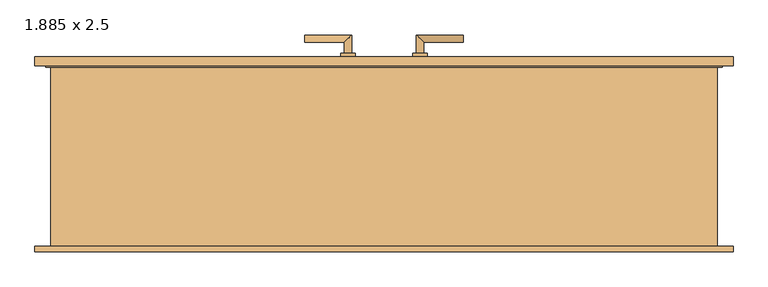
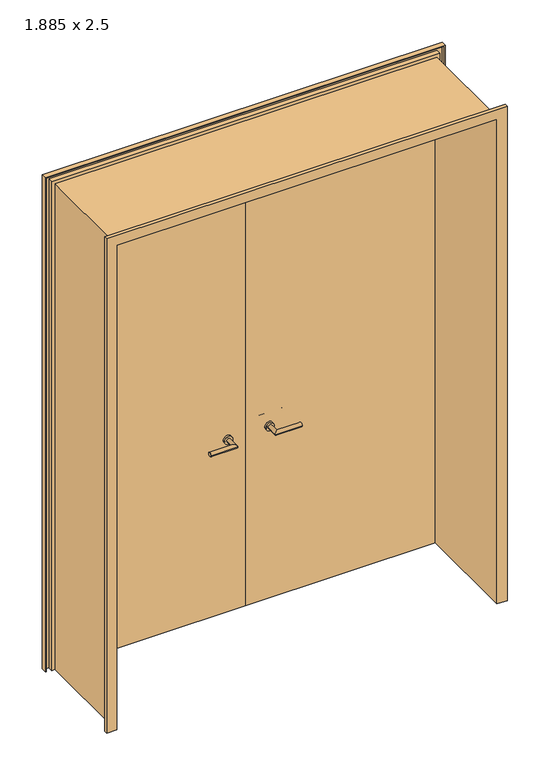
"""IFC4 building model written with IfcOpenShell, lengths in millimetres: door geometry, Drehflügel 2-flg - Stahlzarge : 1.885 x 2.5."""

from ifc_helpers import new_model, si_unit, point, frame, frame_2d, origin, place, context, project, spatial, polyline, circle_curve, ellipse_curve, trimmed, segment, composite_curve, outline, extrude, faceted_brep, source, transform, mapped, element, save
from ifc_brep_helpers import plane_surface, cylinder_surface, advanced_brep


def door_1_885_x_2_5_dd39479c(model_context):
    return source(origin(), model_context, "Body", "SolidModel", [
        advanced_brep(
        [(-90.0, 239.4346141, 901.0), (-110.0, 239.4346141, 901.0), (-110.0, 189.4346141, 901.0), (-90.0, 169.4346141, 901.0), (-220.0, 169.4346141, 901.0), (-220.0, 189.4346141, 901.0)],
        [
            (0, 1, circle_curve(frame((-100.0, 239.4346141, 901.0), z_axis=(0.0, 1.0, 0.0), x_axis=(-1.0, 0.0, 0.0)), 10.0)),
            (1, 0, circle_curve(frame((-100.0, 239.4346141, 901.0), z_axis=(0.0, 1.0, 0.0), x_axis=(-1.0, 0.0, 0.0)), 10.0)),
            (1, 2),
            (2, 3, ellipse_curve(frame((-100.0, 179.4346141, 901.0), z_axis=(0.7071067811865385, 0.7071067811865565, 0.0), x_axis=(-0.7071067811865563, 0.7071067811865386, 0.0)), 14.1421356, 10.0)),
            (3, 0),
            (3, 2, ellipse_curve(frame((-100.0, 179.4346141, 901.0), z_axis=(0.7071067811865385, 0.7071067811865565, 0.0), x_axis=(-0.7071067811865563, 0.7071067811865386, 0.0)), 14.1421356, 10.0)),
            (4, 5, circle_curve(frame((-220.0, 179.4346141, 901.0), z_axis=(-1.0, 0.0, 0.0), x_axis=(0.0, 1.0, 0.0)), 10.0)),
            (5, 4, circle_curve(frame((-220.0, 179.4346141, 901.0), z_axis=(-1.0, 0.0, 0.0), x_axis=(0.0, 1.0, 0.0)), 10.0)),
            (2, 5),
            (4, 3),
        ],
        [
            plane_surface(frame((-100.0, 239.4346141, -386.7526403), z_axis=(0.0, 1.0, 0.0), x_axis=(0.0, 0.0, 1.0))),
            cylinder_surface(frame((-100.0, 239.4346141, 901.0), z_axis=(0.0, 1.0, 0.0), x_axis=(-1.0, 0.0, 0.0)), 10.0),
            plane_surface(frame((-220.0, 179.4346141, -386.7526403), z_axis=(-1.0, 0.0, 0.0), x_axis=(0.0, 0.0, 1.0))),
            cylinder_surface(frame((-100.0, 179.4346141, 901.0), z_axis=(1.0, 0.0, 0.0), x_axis=(0.0, 1.0, 0.0)), 10.0),
        ],
        [
            (0, [[1, 2]]),
            (1, [[3, 4, 5, -2]]),
            (1, [[-5, 6, -3, -1]]),
            (2, [[7, 8]]),
            (3, [[9, -7, 10, -4]]),
            (3, [[-10, -8, -9, -6]]),
        ],
    ),
        advanced_brep(
        [(-110.0, 299.4346141, 901.0), (-90.0, 299.4346141, 901.0), (-90.0, 349.4346141, 901.0), (-110.0, 329.4346141, 901.0), (-220.0, 329.4346141, 901.0), (-220.0, 349.4346141, 901.0)],
        [
            (0, 1, circle_curve(frame((-100.0, 299.4346141, 901.0), z_axis=(0.0, -1.0, 0.0), x_axis=(1.0, 0.0, 0.0)), 10.0)),
            (1, 0, circle_curve(frame((-100.0, 299.4346141, 901.0), z_axis=(0.0, -1.0, 0.0), x_axis=(1.0, 0.0, 0.0)), 10.0)),
            (1, 2),
            (2, 3, ellipse_curve(frame((-100.0, 339.4346141, 901.0), z_axis=(0.7071067811865475, -0.7071067811865475, 0.0), x_axis=(-0.7071067811865474, -0.7071067811865476, 0.0)), 14.1421356, 10.0)),
            (3, 0),
            (3, 2, ellipse_curve(frame((-100.0, 339.4346141, 901.0), z_axis=(0.7071067811865475, -0.7071067811865475, 0.0), x_axis=(-0.7071067811865474, -0.7071067811865476, 0.0)), 14.1421356, 10.0)),
            (4, 5, circle_curve(frame((-220.0, 339.4346141, 901.0), z_axis=(-1.0, 0.0, 0.0), x_axis=(0.0, 1.0, 0.0)), 10.0)),
            (5, 4, circle_curve(frame((-220.0, 339.4346141, 901.0), z_axis=(-1.0, 0.0, 0.0), x_axis=(0.0, 1.0, 0.0)), 10.0)),
            (2, 5),
            (4, 3),
        ],
        [
            plane_surface(frame((-100.0, 299.4346141, -386.7526403), z_axis=(0.0, -1.0, 0.0), x_axis=(0.0, 0.0, 1.0))),
            cylinder_surface(frame((-100.0, 299.4346141, 901.0), z_axis=(0.0, -1.0, 0.0), x_axis=(1.0, 0.0, 0.0)), 10.0),
            plane_surface(frame((-220.0, 339.4346141, -386.7526403), z_axis=(-1.0, 0.0, 0.0), x_axis=(0.0, 0.0, 1.0))),
            cylinder_surface(frame((-100.0, 339.4346141, 901.0), z_axis=(1.0, 0.0, 0.0), x_axis=(0.0, 1.0, 0.0)), 10.0),
        ],
        [
            (0, [[1, 2]]),
            (1, [[3, 4, 5, -2]]),
            (1, [[-5, 6, -3, -1]]),
            (2, [[7, 8]]),
            (3, [[9, -7, 10, -4]]),
            (3, [[-10, -8, -9, -6]]),
        ],
    ),
        extrude(outline(composite_curve([segment(trimmed(circle_curve(frame_2d((901.0, -100.0)), 20.0), [point((901.0, -80.0))], [point((901.0, -120.0))], False, "CARTESIAN"), True, "CONTINUOUS"), segment(trimmed(circle_curve(frame_2d((901.0, -100.0)), 20.0), [point((901.0, -120.0))], [point((901.0, -80.0))], False, "CARTESIAN"), True, "CONTINUOUS")], self_intersect=False)), frame((0.0, 229.4346141, 0.0), z_axis=(0.0, 1.0, 0.0), x_axis=(0.0, 0.0, 1.0)), (0.0, 0.0, 1.0), 10.0),
        extrude(outline(composite_curve([segment(trimmed(circle_curve(frame_2d((901.0, -100.0)), 20.0), [point((901.0, -80.0))], [point((901.0, -120.0))], False, "CARTESIAN"), True, "CONTINUOUS"), segment(trimmed(circle_curve(frame_2d((901.0, -100.0)), 20.0), [point((901.0, -120.0))], [point((901.0, -80.0))], False, "CARTESIAN"), True, "CONTINUOUS")], self_intersect=False)), frame((0.0, 289.4346141, 0.0), z_axis=(0.0, 1.0, 0.0), x_axis=(0.0, 0.0, 1.0)), (0.0, 0.0, 1.0), 10.0),
        advanced_brep(
        [(90.0, 239.4346141, 901.0), (110.0, 239.4346141, 901.0), (90.0, 169.4346141, 901.0), (110.0, 189.4346141, 901.0), (220.0, 169.4346141, 901.0), (220.0, 189.4346141, 901.0)],
        [
            (0, 1, circle_curve(frame((100.0, 239.4346141, 901.0), z_axis=(0.0, 1.0, 0.0), x_axis=(1.0, 0.0, 0.0)), 10.0)),
            (1, 0, circle_curve(frame((100.0, 239.4346141, 901.0), z_axis=(0.0, 1.0, 0.0), x_axis=(1.0, 0.0, 0.0)), 10.0)),
            (0, 2),
            (2, 3, ellipse_curve(frame((100.0, 179.4346141, 901.0), z_axis=(-0.7071067811865385, 0.7071067811865565, 0.0), x_axis=(0.7071067811865563, 0.7071067811865386, 0.0)), 14.1421356, 10.0)),
            (3, 1),
            (3, 2, ellipse_curve(frame((100.0, 179.4346141, 901.0), z_axis=(-0.7071067811865385, 0.7071067811865565, 0.0), x_axis=(0.7071067811865563, 0.7071067811865386, 0.0)), 14.1421356, 10.0)),
            (4, 5, circle_curve(frame((220.0, 179.4346141, 901.0), z_axis=(1.0, 0.0, 0.0), x_axis=(0.0, 1.0, 0.0)), 10.0)),
            (5, 4, circle_curve(frame((220.0, 179.4346141, 901.0), z_axis=(1.0, 0.0, 0.0), x_axis=(0.0, 1.0, 0.0)), 10.0)),
            (2, 4),
            (5, 3),
        ],
        [
            plane_surface(frame((100.0, 239.4346141, -386.7526403), z_axis=(0.0, 1.0, 0.0), x_axis=(0.0, 0.0, 1.0))),
            cylinder_surface(frame((100.0, 239.4346141, 901.0), z_axis=(0.0, 1.0, 0.0), x_axis=(1.0, 0.0, 0.0)), 10.0),
            plane_surface(frame((220.0, 179.4346141, -386.7526403), z_axis=(1.0, 0.0, 0.0), x_axis=(0.0, 0.0, 1.0))),
            cylinder_surface(frame((100.0, 179.4346141, 901.0), z_axis=(-1.0, 0.0, 0.0), x_axis=(0.0, 1.0, 0.0)), 10.0),
        ],
        [
            (0, [[1, 2]]),
            (1, [[-1, 3, 4, 5]]),
            (1, [[-2, -5, 6, -3]]),
            (2, [[7, 8]]),
            (3, [[-4, 9, -8, 10]]),
            (3, [[-6, -10, -7, -9]]),
        ],
    ),
        advanced_brep(
        [(110.0, 299.4346141, 901.0), (90.0, 299.4346141, 901.0), (110.0, 329.4346141, 901.0), (90.0, 349.4346141, 901.0), (220.0, 329.4346141, 901.0), (220.0, 349.4346141, 901.0)],
        [
            (0, 1, circle_curve(frame((100.0, 299.4346141, 901.0), z_axis=(0.0, -1.0, 0.0), x_axis=(-1.0, 0.0, 0.0)), 10.0)),
            (1, 0, circle_curve(frame((100.0, 299.4346141, 901.0), z_axis=(0.0, -1.0, 0.0), x_axis=(-1.0, 0.0, 0.0)), 10.0)),
            (0, 2),
            (2, 3, ellipse_curve(frame((100.0, 339.4346141, 901.0), z_axis=(-0.7071067811865475, -0.7071067811865475, 0.0), x_axis=(0.7071067811865474, -0.7071067811865476, 0.0)), 14.1421356, 10.0)),
            (3, 1),
            (3, 2, ellipse_curve(frame((100.0, 339.4346141, 901.0), z_axis=(-0.7071067811865475, -0.7071067811865475, 0.0), x_axis=(0.7071067811865474, -0.7071067811865476, 0.0)), 14.1421356, 10.0)),
            (4, 5, circle_curve(frame((220.0, 339.4346141, 901.0), z_axis=(1.0, 0.0, 0.0), x_axis=(0.0, 1.0, 0.0)), 10.0)),
            (5, 4, circle_curve(frame((220.0, 339.4346141, 901.0), z_axis=(1.0, 0.0, 0.0), x_axis=(0.0, 1.0, 0.0)), 10.0)),
            (2, 4),
            (5, 3),
        ],
        [
            plane_surface(frame((100.0, 299.4346141, -386.7526403), z_axis=(0.0, -1.0, 0.0), x_axis=(0.0, 0.0, 1.0))),
            cylinder_surface(frame((100.0, 299.4346141, 901.0), z_axis=(0.0, -1.0, 0.0), x_axis=(-1.0, 0.0, 0.0)), 10.0),
            plane_surface(frame((220.0, 339.4346141, -386.7526403), z_axis=(1.0, 0.0, 0.0), x_axis=(0.0, 0.0, 1.0))),
            cylinder_surface(frame((100.0, 339.4346141, 901.0), z_axis=(-1.0, 0.0, 0.0), x_axis=(0.0, 1.0, 0.0)), 10.0),
        ],
        [
            (0, [[1, 2]]),
            (1, [[-1, 3, 4, 5]]),
            (1, [[-2, -5, 6, -3]]),
            (2, [[7, 8]]),
            (3, [[-4, 9, -8, 10]]),
            (3, [[-6, -10, -7, -9]]),
        ],
    ),
        extrude(outline(composite_curve([segment(trimmed(circle_curve(frame_2d((901.0, 100.0)), 20.0), [point((901.0, 80.0))], [point((901.0, 120.0))], False, "CARTESIAN"), True, "CONTINUOUS"), segment(trimmed(circle_curve(frame_2d((901.0, 100.0)), 20.0), [point((901.0, 120.0))], [point((901.0, 80.0))], False, "CARTESIAN"), True, "CONTINUOUS")], self_intersect=False)), frame((0.0, 229.4346141, 0.0), z_axis=(0.0, 1.0, 0.0), x_axis=(0.0, 0.0, 1.0)), (0.0, 0.0, 1.0), 10.0),
        extrude(outline(composite_curve([segment(trimmed(circle_curve(frame_2d((901.0, 100.0)), 20.0), [point((901.0, 80.0))], [point((901.0, 120.0))], False, "CARTESIAN"), True, "CONTINUOUS"), segment(trimmed(circle_curve(frame_2d((901.0, 100.0)), 20.0), [point((901.0, 120.0))], [point((901.0, 80.0))], False, "CARTESIAN"), True, "CONTINUOUS")], self_intersect=False)), frame((0.0, 289.4346141, 0.0), z_axis=(0.0, 1.0, 0.0), x_axis=(0.0, 0.0, 1.0)), (0.0, 0.0, 1.0), 10.0),
        extrude(outline(polyline([(0.0, 264.4346141), (-932.5, 264.4346141), (-932.5, 289.4346141), (0.0, 289.4346141), (0.0, 264.4346141)])), frame((0.0, 0.0, 1.0), z_axis=(0.0, 0.0, 1.0), x_axis=(1.0, 0.0, 0.0)), (0.0, 0.0, 1.0), 2490.0),
        extrude(outline(polyline([(932.5, 264.4346141), (0.0, 264.4346141), (0.0, 289.4346141), (932.5, 289.4346141), (932.5, 264.4346141)])), frame((0.0, 0.0, 1.0), z_axis=(0.0, 0.0, 1.0), x_axis=(1.0, 0.0, 0.0)), (0.0, 0.0, 1.0), 2490.0),
        faceted_brep([(967.0, -250.5653859, 1.0), (917.5, -250.5653859, 1.0), (917.5, 264.4346141, 1.0), (932.5, 264.4346141, 1.0), (932.5, 289.4346141, 1.0), (967.0, 289.4346141, 1.0), (967.0, 264.4346141, 1.0), (962.0, 264.4346141, 1.0), (962.0, 284.4346141, 1.0), (937.5, 284.4346141, 1.0), (937.5, 259.4346141, 1.0), (922.5, 259.4346141, 1.0), (922.5, -245.5653859, 1.0), (962.0, -245.5653859, 1.0), (962.0, -235.5653859, 1.0), (967.0, -235.5653859, 1.0), (967.0, -250.5653859, 2525.5), (-967.0, -250.5653859, 2525.5), (-967.0, -250.5653859, 1.0), (-917.5, -250.5653859, 1.0), (-917.5, -250.5653859, 2476.0), (917.5, -250.5653859, 2476.0), (917.5, 264.4346141, 2476.0), (-917.5, 264.4346141, 2476.0), (-917.5, 264.4346141, 1.0), (-932.5, 264.4346141, 1.0), (-932.5, 264.4346141, 2491.0), (932.5, 264.4346141, 2491.0), (932.5, 289.4346141, 2491.0), (-932.5, 289.4346141, 2491.0), (-932.5, 289.4346141, 1.0), (-967.0, 289.4346141, 1.0), (-967.0, 289.4346141, 2525.5), (967.0, 289.4346141, 2525.5), (967.0, 264.4346141, 2525.5), (-967.0, 264.4346141, 2525.5), (-967.0, 264.4346141, 1.0), (-962.0, 264.4346141, 1.0), (-962.0, 264.4346141, 2520.5), (962.0, 264.4346141, 2520.5), (962.0, 284.4346141, 2520.5), (-962.0, 284.4346141, 2520.5), (-962.0, 284.4346141, 1.0), (-937.5, 284.4346141, 1.0), (-937.5, 284.4346141, 2496.0), (937.5, 284.4346141, 2496.0), (937.5, 259.4346141, 2496.0), (-937.5, 259.4346141, 2496.0), (-937.5, 259.4346141, 1.0), (-922.5, 259.4346141, 1.0), (-922.5, 259.4346141, 2481.0), (922.5, 259.4346141, 2481.0), (922.5, -245.5653859, 2481.0), (-922.5, -245.5653859, 2481.0), (-922.5, -245.5653859, 1.0), (-962.0, -245.5653859, 1.0), (-962.0, -245.5653859, 2520.5), (962.0, -245.5653859, 2520.5), (962.0, -235.5653859, 2520.5), (-962.0, -235.5653859, 2520.5), (-962.0, -235.5653859, 1.0), (-967.0, -235.5653859, 1.0), (-967.0, -235.5653859, 2525.5), (967.0, -235.5653859, 2525.5)], [[[0, 1, 2, 3, 4, 5, 6, 7, 8, 9, 10, 11, 12, 13, 14, 15]], [[1, 0, 16, 17, 18, 19, 20, 21]], [[2, 1, 21, 22]], [[3, 2, 22, 23, 24, 25, 26, 27]], [[4, 3, 27, 28]], [[5, 4, 28, 29, 30, 31, 32, 33]], [[6, 5, 33, 34]], [[7, 6, 34, 35, 36, 37, 38, 39]], [[8, 7, 39, 40]], [[9, 8, 40, 41, 42, 43, 44, 45]], [[10, 9, 45, 46]], [[11, 10, 46, 47, 48, 49, 50, 51]], [[12, 11, 51, 52]], [[13, 12, 52, 53, 54, 55, 56, 57]], [[14, 13, 57, 58]], [[15, 14, 58, 59, 60, 61, 62, 63]], [[0, 15, 63, 16]], [[17, 62, 61, 18]], [[18, 61, 60, 55, 54, 49, 48, 43, 42, 37, 36, 31, 30, 25, 24, 19]], [[23, 20, 19, 24]], [[29, 26, 25, 30]], [[35, 32, 31, 36]], [[41, 38, 37, 42]], [[47, 44, 43, 48]], [[53, 50, 49, 54]], [[59, 56, 55, 60]], [[22, 21, 20, 23]], [[28, 27, 26, 29]], [[34, 33, 32, 35]], [[40, 39, 38, 41]], [[46, 45, 44, 47]], [[52, 51, 50, 53]], [[58, 57, 56, 59]], [[16, 63, 62, 17]]]),
    ])


if __name__ == "__main__":
    model = new_model("IFC4")
    model_context = context("Model", 3, world=origin())
    ifc_project = project(units=[si_unit("LENGTHUNIT", "METRE", prefix="MILLI")], contexts=[model_context])
    site = spatial("IfcSite", under=ifc_project)
    building = spatial("IfcBuilding", under=site)
    placement = place(None, origin())
    door_1_885_x_2_5_shape = door_1_885_x_2_5_dd39479c(model_context)
    element("IfcDoor", 1, ObjectType="Drehflügel 2-flg - Stahlzarge : 1.885 x 2.5", at=placement, inside=building, context=model_context, shape_type="MappedRepresentation", body=[
        mapped(door_1_885_x_2_5_shape, transform((0.0, 0.0, 0.0), x_axis=(1.0, 0.0, 0.0), y_axis=(0.0, 1.0, 0.0), z_axis=(0.0, 0.0, 1.0))),
    ])
    save(model, "model.ifc")

# Revit data of these elements
# Type "Drehflügel 2-flg - Stahlzarge : 1.885 x 2.5"
#   Type Mark = "23"
#   Construction Type Id = "MDOOR"
#   Operation = "DoubleDoorSingleSwing"
#   Keynote = "16.03"
#   Analytic Construction = "Metall"
#   Heat Transfer Coefficient (U) = 3.7021 W/(m²·K)
#   Rough Width = 1.885 m
#   Rough Height [instance default] = 2.600 m
#   Höhe Türgriff = 0.900 m
#   Height = 2.500 m
#   Fußbodenaufbau [instance default] = 0.100 m
#   Width = 1.885 m
#   Sichtbarkeit Sturzlinien [instance default] = yes
#   Türgriff auswählen [instance default] = element 219327
#   Türgriff [instance default] = none
#   Türflügel [instance default] = none
#   Rahmen/Pfosten [instance default] = Metall - Lackiert - Grau
#   Visual Light Transmittance = 0
#   Solar Heat Gain Coefficient = 0
#   Function = (empty or 0)
#   Wall Closure = (empty or 0)
# Element 1 (IfcDoor, "Drehflügel 2-flg - Stahlzarge : 1.885 x 2.5")
#   Rough Height = 2.501 m
#   Fußbodenaufbau = 0.001 m
#   Materials on its faces: "Metall - Chrom", "Metall - Lackiert - Grau", "Holz - Birke"
# Materials
#   "Metall - Lackiert - Grau": class "Farbe 1", colour RGB 98 98 98, transparency 0, Cost = 0
#   "Metall - Chrom": class "Metall", colour RGB 247 247 247, transparency 0, Cost = 0
#   "Holz - Birke": class "Holz", colour RGB 213 164 103, transparency 0, Cost = 0
